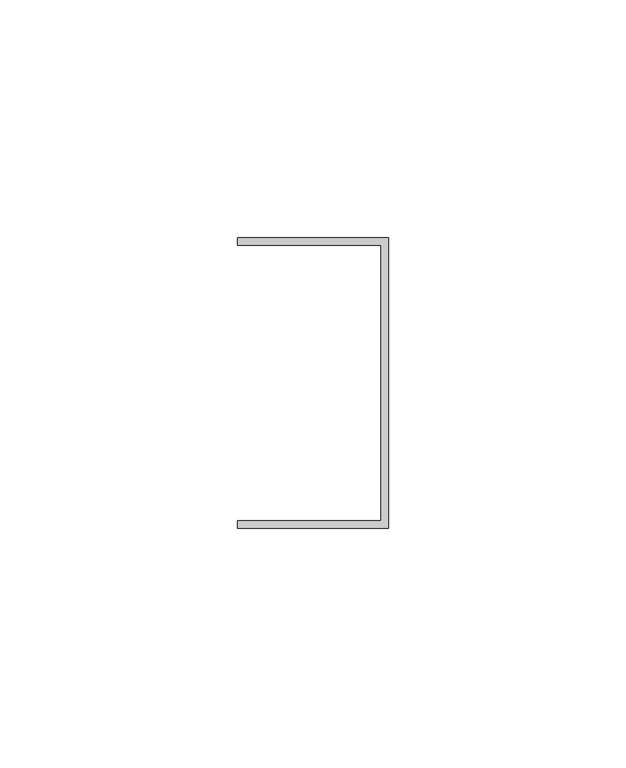
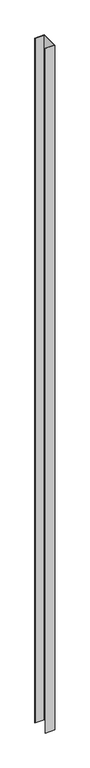
"""IFC4 building model written with IfcOpenShell, lengths in millimetres: proxy geometry, Generic Models 7:Generic Models 1:3:Generic Models 1:3 : Generic Models 7:Generic Models 1:305549:3:Generic Models 1:3:Generic Models 1:3 : Generic Models 7:Generic Models 1:305549:3 : Generic Models 7:Generic Models 1:3:Generic Models 1:3 : Generic Models 7:Generic Models 1:305549:301244:25 : Generic Models 7:Generic Models 1:3:Generic Models 1:3 : Generic Models 7:Generic Models 1:305549:3:Generic Models 1:3:Generic Models 1:3 : Generic Models 7:Generic Models 1:305549:3 : Generic Models 7:Generic Models 1:3:Generic Models 1:3 : Generic Models 7:Generic Models 1:305549:301244:308848."""

from ifc_helpers import new_model, si_unit, frame, origin, place, context, project, spatial, polyline, outline, extrude, source, transform, mapped, element, save


def generic_models_f29e4c72(model_context):
    return source(origin(), model_context, "Body", "SweptSolid", [
        extrude(outline(polyline([(579069.586724, -579015.772634), (579069.586724, -579076.8913841), (579037.836724, -579076.8913841), (579037.836724, -579075.3038841), (579067.999224, -579075.3038841), (579067.999224, -579017.360134), (579037.836724, -579017.360134), (579037.836724, -579015.772634), (579069.586724, -579015.772634)])), frame((0.0, 0.0, 3721.1), z_axis=(0.0, 0.0, 1.0), x_axis=(1.0, 0.0, 0.0)), (0.0, 0.0, 1.0), 2430.9324376),
    ])


if __name__ == "__main__":
    model = new_model("IFC4")
    model_context = context("Model", 3, world=origin())
    ifc_project = project(units=[si_unit("LENGTHUNIT", "METRE", prefix="MILLI")], contexts=[model_context])
    site = spatial("IfcSite", under=ifc_project)
    building = spatial("IfcBuilding", under=site)
    placement = place(None, origin())
    generic_models_shape = generic_models_f29e4c72(model_context)
    element("IfcBuildingElementProxy", 1, Name="Generic Models 7:Generic Models 1:3:Generic Models 1:3 : Generic Models 7:Generic Models 1:305549:3:Generic Models 1:3:Generic Models 1:3 : Generic Models 7:Generic Models 1:305549:3 : Generic Models 7:Generic Models 1:3:Generic Models 1:3 : Generic Models 7:Generic Models 1:305549:301244:25 : Generic Models 7:Generic Models 1:3:Generic Models 1:3 : Generic Models 7:Generic Models 1:305549:3:Generic Models 1:3:Generic Models 1:3 : Generic Models 7:Generic Models 1:305549:3 : Generic Models 7:Generic Models 1:3:Generic Models 1:3 : Generic Models 7:Generic Models 1:305549:301244:308848", ObjectType="Generic Models 7:Generic Models 1:3:Generic Models 1:3 : Generic Models 7:Generic Models 1:305549:3:Generic Models 1:3:Generic Models 1:3 : Generic Models 7:Generic Models 1:305549:3 : Generic Models 7:Generic Models 1:3:Generic Models 1:3 : Generic Models 7:Generic Models 1:305549:301244:25 : Generic Models 7:Generic Models 1:3:Generic Models 1:3 : Generic Models 7:Generic Models 1:305549:3:Generic Models 1:3:Generic Models 1:3 : Generic Models 7:Generic Models 1:305549:3 : Generic Models 7:Generic Models 1:3:Generic Models 1:3 : Generic Models 7:Generic Models 1:305549:301244:308848", at=placement, inside=building, context=model_context, shape_type="MappedRepresentation", body=[
        mapped(generic_models_shape, transform((0.0, 0.0, 0.0), x_axis=(1.0, 0.0, 0.0), y_axis=(0.0, 1.0, 0.0), z_axis=(0.0, 0.0, 1.0))),
    ])
    save(model, "model.ifc")

# Revit data of these elements
# Type "Generic Models 7:Generic Models 1:3:Generic Models 1:3 : Generic Models 7:Generic Models 1:305549:3:Generic Models 1:3:Generic Models 1:3 : Generic Models 7:Generic Models 1:305549:3 : Generic Models 7:Generic Models 1:3:Generic Models 1:3 : Generic Models 7:Generic Models 1:305549:301244:25 : Generic Models 7:Generic Models 1:3:Generic Models 1:3 : Generic Models 7:Generic Models 1:305549:3:Generic Models 1:3:Generic Models 1:3 : Generic Models 7:Generic Models 1:305549:3 : Generic Models 7:Generic Models 1:3:Generic Models 1:3 : Generic Models 7:Generic Models 1:305549:301244:308848"
#   NameOverride = "Generic Models 7:Generic Models 1:3:Generic Models 1:3 : Generic Models 7:Generic Models 1:305549:3:Generic Models 1:3:Generic Models 1:3 : Generic Models 7:Generic Models 1:305549:3 : Generic Models 7:Generic Models 1:3:Generic Models 1:3 : Generic Models 7:Generic Models 1:305549:301244:308848"
#   ObjectTypeOverride = "Generic Models 1:3:Generic Models 1:3 : Generic Models 7:Generic Models 1:305549:3 : Generic Models 7:Generic Models 1:3:Generic Models 1:3 : Generic Models 7:Generic Models 1:305549:301244"
#   Reference = "Generic Models 1"
#   Tag = "308848"
# Element 1 (IfcBuildingElementProxy, "Generic Models 7:Generic Models 1:3:Generic Models 1:3 : Generic Models 7:Generic Models 1:305549:3:Generic Models 1:3:Generic Models 1:3 : Generic Models 7:Generic Models 1:305549:3 : Generic Models 7:Generic Models 1:3:Generic Models 1:3 : Generic Models 7:Generic Models 1:305549:301244:25 : Generic Models 7:Generic Models 1:3:Generic Models 1:3 : Generic Models 7:Generic Models 1:305549:3:Generic Models 1:3:Generic Models 1:3 : Generic Models 7:Generic Models 1:305549:3 : Generic Models 7:Generic Models 1:3:Generic Models 1:3 : Generic Models 7:Generic Models 1:305549:301244:308848")
#   Materials on its faces: "GALVANIZED U-CHANNEL (250T125-33)"
# Materials
#   "GALVANIZED U-CHANNEL (250T125-33)": class "Unassigned", colour RGB 202 201 200, transparency 0, Keynote = "M05451300.02", Cost = 0
